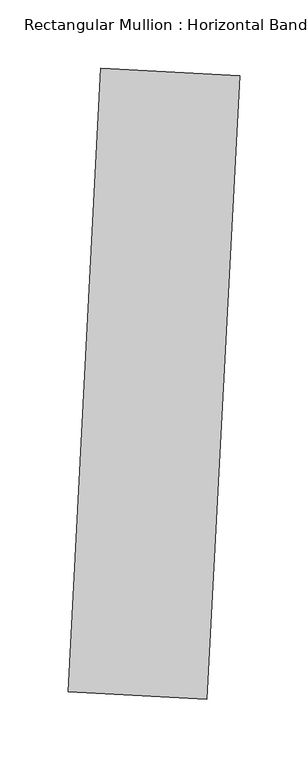
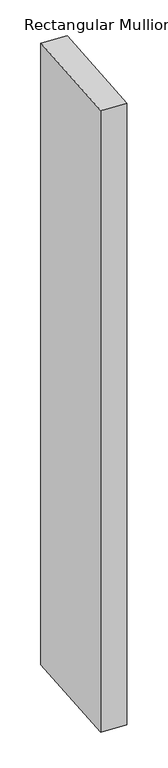
"""IFC4 building model written with IfcOpenShell, lengths in millimetres: member geometry, Rectangular Mullion : Horizontal Band."""

from ifc_helpers import new_model, si_unit, frame, origin, place, context, project, spatial, polyline, outline, extrude, source, transform, mapped, element, save


def rectangular_mullion_horizontal_band_87718f43(model_context):
    return source(origin(), model_context, "Body", "SweptSolid", [
        extrude(outline(polyline([(62.69438, 301.8280451), (38.7663808, -154.7453782), (-62.69438, -149.4280451), (-38.7663808, 307.1453782), (62.69438, 301.8280451)])), frame((0.0, 0.0, -2629.1291719), z_axis=(0.0, 0.0, 1.0), x_axis=(1.0, 0.0, 0.0)), (0.0, 0.0, 1.0), 2629.1291719),
    ])


if __name__ == "__main__":
    model = new_model("IFC4")
    model_context = context("Model", 3, world=origin())
    ifc_project = project(units=[si_unit("LENGTHUNIT", "METRE", prefix="MILLI")], contexts=[model_context])
    site = spatial("IfcSite", under=ifc_project)
    building = spatial("IfcBuilding", under=site)
    placement = place(None, origin())
    rectangular_mullion_horizontal_band_shape = rectangular_mullion_horizontal_band_87718f43(model_context)
    element("IfcMember", 1, ObjectType="Rectangular Mullion : Horizontal Band", at=placement, inside=building, context=model_context, shape_type="MappedRepresentation", body=[
        mapped(rectangular_mullion_horizontal_band_shape, transform((0.0, 0.0, 0.0), x_axis=(1.0, 0.0, 0.0), y_axis=(0.0, 1.0, 0.0), z_axis=(0.0, 0.0, 1.0))),
    ])
    save(model, "model.ifc")

# Revit data of these elements
# Type "Rectangular Mullion : Horizontal Band"
#   built-in parameter 1007351 = 0.25 (stored number, unit not read)
#   built-in parameter 1007304 = 1.5 (stored number, unit not read)
#   built-in parameter 1007301 = 0.166667 (stored number, unit not read)
#   built-in parameter 1007300 = 0.166667 (stored number, unit not read)
# Element 1 (IfcMember, "Rectangular Mullion : Horizontal Band")
#   Materials on its faces: "Aluminum"
# Materials
#   "Aluminum": class "Metal", colour RGB 247 247 247, transparency 0, Description = "Aluminum 6061", Cost = 0
